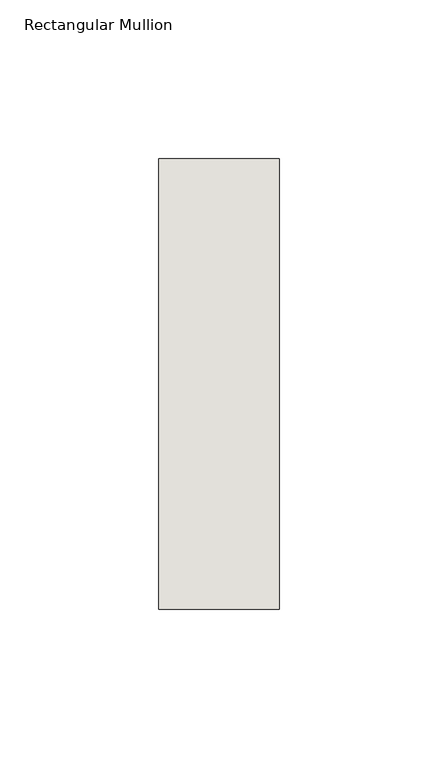
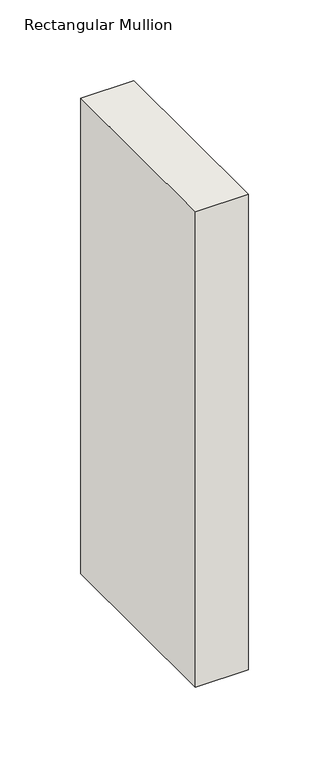
"""IFC4 building model written with IfcOpenShell, lengths in millimetres: wall geometry, Rectangular Mullion : NLRS_21_CWM_hsb-regel 38x142_gen_rsf."""

from ifc_helpers import new_model, si_unit, frame, origin, place, context, project, spatial, polyline, outline, extrude, source, transform, mapped, element, save


def rectangular_mullion_ee68c600(model_context):
    return source(origin(), model_context, "Body", "SweptSolid", [
        extrude(outline(polyline([(-38.0, -71.0), (-38.0, 71.0), (0.0, 71.0), (0.0, -71.0), (-38.0, -71.0)])), frame((0.0, 0.0, -359.9999997), z_axis=(0.0, 0.0, 1.0), x_axis=(1.0, 0.0, 0.0)), (0.0, 0.0, 1.0), 359.9999997),
    ])


if __name__ == "__main__":
    model = new_model("IFC4")
    model_context = context("Model", 3, world=origin())
    ifc_project = project(units=[si_unit("LENGTHUNIT", "METRE", prefix="MILLI")], contexts=[model_context])
    site = spatial("IfcSite", under=ifc_project)
    building = spatial("IfcBuilding", under=site)
    placement = place(None, origin())
    rectangular_mullion_shape = rectangular_mullion_ee68c600(model_context)
    element("IfcWall", 1, ObjectType="Rectangular Mullion : NLRS_21_CWM_hsb-regel 38x142_gen_rsf", at=placement, inside=building, context=model_context, shape_type="MappedRepresentation", body=[
        mapped(rectangular_mullion_shape, transform((0.0, 0.0, 0.0), x_axis=(1.0, 0.0, 0.0), y_axis=(0.0, 1.0, 0.0), z_axis=(0.0, 0.0, 1.0))),
    ])
    save(model, "model.ifc")

# Revit data of these elements
# Type "Rectangular Mullion : NLRS_21_CWM_hsb-regel 38x142_gen_rsf"
#   Type IfcGUID = "07M7mRoiH1CR8m_RSKIwpF"
#   Assembly Code = "21.10"
#   IfcExportAs = "IfcWall"
#   built-in parameter 1007322 = 0.465879 (stored number, unit not read)
#   built-in parameter 1007321 = 0.062336 (stored number, unit not read)
#   built-in parameter 1007320 = 0.062336 (stored number, unit not read)
# Element 1 (IfcWall, "Rectangular Mullion : NLRS_21_CWM_hsb-regel 38x142_gen_rsf")
#   Materials on its faces: "NLRS_i2_hout naaldhout vuren_gen_rsf"
# Materials
#   "NLRS_i2_hout naaldhout vuren_gen_rsf": class "I - Hout", colour RGB 234 199 147, transparency 0, Keynote = "i2", Manufacturer = "Revit Standards Foundation", URL = "www.revitstandards.org", Description = "hout vuren", Cost = 0
